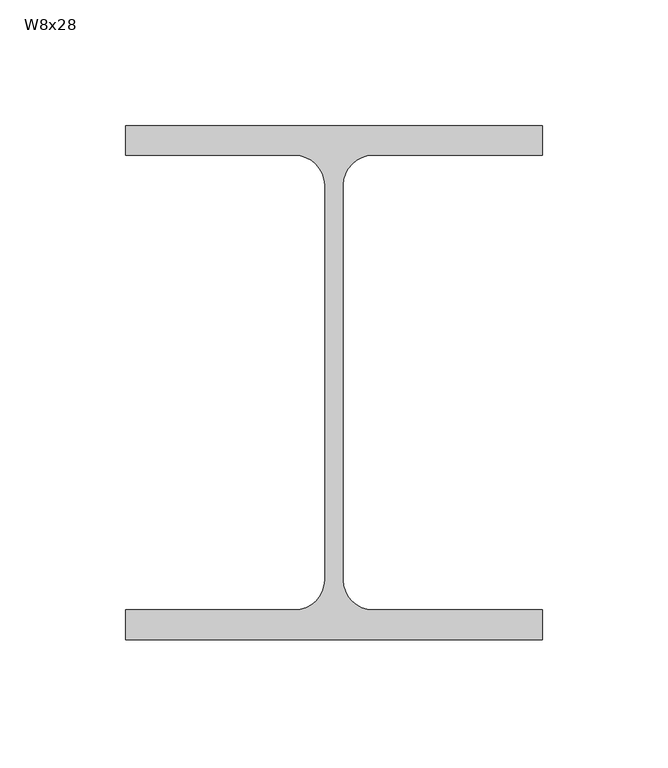
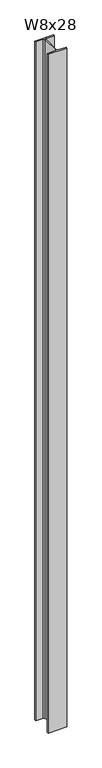
"""IFC4 building model written with IfcOpenShell, lengths in millimetres: column geometry, RME WF - Column : W8x28."""

import ifcopenshell
import ifcopenshell.guid

model = None  # the IFC model being written
_history = None  # IfcOwnerHistory: only IFC2X3 demands one
_inside = {}  # id of a spatial element -> (the spatial element, [elements in it])
_under = {}  # id of a project, library or spatial element -> (it, [spatial elements below it])
_declared = {}  # id of a project -> (the project, [libraries it declares])
_typed = {}  # id of a type object -> (the type object, [elements of that type])
_made_of = {}  # id of a material, layer set ... -> (it, [elements and type objects made of it])


def new_model(schema):
    """Start an empty IFC model of exactly this schema.

    Asked for "IFC4X3", IfcOpenShell would pick the latest addendum, in which some entities
    have other attributes; the version numbers below select the first issue.
    IFC2X3 requires an IfcOwnerHistory on every rooted entity: one is made here for all.
    """
    global model, _history
    if schema == "IFC4X3":
        model = ifcopenshell.file(schema_version=(4, 3, 0, 0))
    else:
        model = ifcopenshell.file(schema=schema)
    _inside.clear()
    _under.clear()
    _declared.clear()
    _typed.clear()
    _made_of.clear()
    _history = None
    if model.schema == "IFC2X3":
        org = make("IfcOrganization", Name="unknown")
        user = make(
            "IfcPersonAndOrganization",
            ThePerson=make("IfcPerson", FamilyName="unknown"),
            TheOrganization=org,
        )
        app = make(
            "IfcApplication",
            ApplicationDeveloper=org,
            Version="unknown",
            ApplicationFullName="unknown",
            ApplicationIdentifier="unknown",
        )
        _history = make(
            "IfcOwnerHistory",
            OwningUser=user,
            OwningApplication=app,
            ChangeAction="ADDED",
            CreationDate=0,
        )
    return model


def make(cls, **values):
    """One entity of the class cls with the attributes given. An attribute that is None is left unset."""
    return model.create_entity(
        cls, **{name: value for name, value in values.items() if value is not None}
    )


def rooted(cls, **values):
    """An entity with a GlobalId (a new one), such as an element, a storey or a relation."""
    return make(cls, GlobalId=ifcopenshell.guid.new(), OwnerHistory=_history, **values)


def si_unit(unit_type, name, prefix=None):
    """IfcSIUnit, for example si_unit("LENGTHUNIT", "METRE", prefix="MILLI")."""
    return make("IfcSIUnit", UnitType=unit_type, Prefix=prefix, Name=name)


def assignment(units):
    """IfcUnitAssignment: the units of a project."""
    return None if units is None else make("IfcUnitAssignment", Units=units)


def point(xyz):
    """IfcCartesianPoint."""
    return None if xyz is None else make("IfcCartesianPoint", Coordinates=xyz)


def direction(xyz):
    """IfcDirection."""
    return None if xyz is None else make("IfcDirection", DirectionRatios=xyz)


def frame(location, z_axis=None, x_axis=None):
    """IfcAxis2Placement3D, a coordinate frame: its origin and axes. An axis left out is left unset."""
    return make(
        "IfcAxis2Placement3D",
        Location=point(location),
        Axis=direction(z_axis),
        RefDirection=direction(x_axis),
    )


def frame_2d(location, x_axis=None):
    """IfcAxis2Placement2D, a coordinate frame in the plane: its origin and x axis."""
    return make(
        "IfcAxis2Placement2D", Location=point(location), RefDirection=direction(x_axis)
    )


def origin():
    """The frame at (0, 0, 0) with its axes left unset."""
    return frame((0.0, 0.0, 0.0))


def place(relative_to, where):
    """IfcLocalPlacement: puts the frame where relative to a parent placement (None: the world)."""
    return make(
        "IfcLocalPlacement", PlacementRelTo=relative_to, RelativePlacement=where
    )


def context(
    kind, dimensions, precision=None, world=None, true_north=None, identifier=None
):
    """IfcGeometricRepresentationContext, for example the 3D "Model" context."""
    return make(
        "IfcGeometricRepresentationContext",
        ContextIdentifier=identifier,
        ContextType=kind,
        CoordinateSpaceDimension=dimensions,
        Precision=precision,
        WorldCoordinateSystem=world,
        TrueNorth=true_north,
    )


def project(units=None, contexts=None):
    """IfcProject with its units and contexts."""
    return rooted(
        "IfcProject",
        Name="project",
        RepresentationContexts=contexts,
        UnitsInContext=assignment(units),
    )


def spatial(cls, under=None, at=None, **own):
    """A site, building, storey or space (cls), placed at a placement, below another one or the project."""
    s = rooted(cls, ObjectPlacement=at, **own)
    if under is not None:
        _under.setdefault(under.id(), (under, []))[1].append(s)
    return s


def polyline(points):
    """IfcPolyline through the points."""
    return make("IfcPolyline", Points=[point(p) for p in points])


def circle_curve(where, radius):
    """IfcCircle in the frame where."""
    return make("IfcCircle", Position=where, Radius=radius)


def trimmed(basis, trim1, trim2, sense, master):
    """IfcTrimmedCurve: the piece of a basis curve between two trims."""
    return make(
        "IfcTrimmedCurve",
        BasisCurve=basis,
        Trim1=trim1,
        Trim2=trim2,
        SenseAgreement=sense,
        MasterRepresentation=master,
    )


def segment(curve, same_sense, transition):
    """IfcCompositeCurveSegment."""
    return make(
        "IfcCompositeCurveSegment",
        Transition=transition,
        SameSense=same_sense,
        ParentCurve=curve,
    )


def composite_curve(segments, self_intersect=None):
    """IfcCompositeCurve: segments joined end to end."""
    return make("IfcCompositeCurve", Segments=segments, SelfIntersect=self_intersect)


def outline(outer, holes=None, kind="AREA"):
    """IfcArbitraryClosedProfileDef: a profile drawn as a closed curve; with holes, ...WithVoids."""
    if holes is None:
        return make("IfcArbitraryClosedProfileDef", ProfileType=kind, OuterCurve=outer)
    return make(
        "IfcArbitraryProfileDefWithVoids",
        ProfileType=kind,
        OuterCurve=outer,
        InnerCurves=holes,
    )


def extrude(swept, where, along, depth):
    """IfcExtrudedAreaSolid: the profile swept, set in the frame where, extruded along a direction by depth."""
    return make(
        "IfcExtrudedAreaSolid",
        SweptArea=swept,
        Position=where,
        ExtrudedDirection=direction(along),
        Depth=depth,
    )


def shape(context_of_items, identifier, shape_type, items):
    """IfcShapeRepresentation: the items that make up one representation, for example the "Body"."""
    return make(
        "IfcShapeRepresentation",
        ContextOfItems=context_of_items,
        RepresentationIdentifier=identifier,
        RepresentationType=shape_type,
        Items=items,
    )


def source(mapping_origin, context_of_items, identifier, shape_type, items):
    """IfcRepresentationMap: a shape defined once, which mapped items show again and again."""
    return make(
        "IfcRepresentationMap",
        MappingOrigin=mapping_origin,
        MappedRepresentation=shape(context_of_items, identifier, shape_type, items),
    )


def transform(
    local_origin,
    x_axis=None,
    y_axis=None,
    z_axis=None,
    scale=None,
    scale2=None,
    scale3=None,
    uniform=True,
):
    """IfcCartesianTransformationOperator3D, or its non-uniform kind. x_axis, y_axis, z_axis: its Axis1, 2, 3."""
    if uniform:
        return make(
            "IfcCartesianTransformationOperator3D",
            Axis1=direction(x_axis),
            Axis2=direction(y_axis),
            LocalOrigin=point(local_origin),
            Scale=scale,
            Axis3=direction(z_axis),
        )
    return make(
        "IfcCartesianTransformationOperator3DnonUniform",
        Axis1=direction(x_axis),
        Axis2=direction(y_axis),
        LocalOrigin=point(local_origin),
        Scale=scale,
        Axis3=direction(z_axis),
        Scale2=scale2,
        Scale3=scale3,
    )


def mapped(mapping_source, mapping_target):
    """IfcMappedItem: shows the shape of a source again, moved by a transform."""
    return make(
        "IfcMappedItem", MappingSource=mapping_source, MappingTarget=mapping_target
    )


def made_of(thing, what):
    """Note that an element or type object is made of a material, layer set ...; save() writes the relation."""
    if what is not None:
        _made_of.setdefault(what.id(), (what, []))[1].append(thing)
    return thing


def element(
    cls,
    number,
    at=None,
    inside=None,
    cuts=None,
    type_object=None,
    material=None,
    context=None,
    identifier="Body",
    shape_type=None,
    held_by="IfcProductDefinitionShape",
    body=None,
    shapes=None,
    **own,
):
    """One element of the class cls, such as IfcWall. Its Tag is "e" and its number.

    at: its placement. inside: the storey or other place that contains it. cuts: it is an
    opening in that element (IfcRelVoidsElement). A single representation is given by context,
    identifier, shape_type and body (its items); several are given by shapes. held_by: the class
    of the entity that holds the representations. save() writes the other relations.
    """
    e = rooted(cls, Tag="e%d" % number, ObjectPlacement=at, **own)
    if body is not None:
        shapes = [shape(context, identifier, shape_type, body)]
    if shapes is not None:
        e.Representation = make(held_by, Representations=shapes)
    if inside is not None:
        _inside.setdefault(inside.id(), (inside, []))[1].append(e)
    if cuts is not None:
        rooted(
            "IfcRelVoidsElement", RelatingBuildingElement=cuts, RelatedOpeningElement=e
        )
    if type_object is not None:
        _typed.setdefault(type_object.id(), (type_object, []))[1].append(e)
    return made_of(e, material)


def aggregate(whole, parts):
    """IfcRelAggregates: a whole, such as a stair, and the parts it consists of."""
    return rooted("IfcRelAggregates", RelatingObject=whole, RelatedObjects=parts)


def save(model, path):
    """Write the relations noted so far, then the file.

    IfcRelAggregates (storeys below a building ...), IfcRelContainedInSpatialStructure (elements
    in a storey), IfcRelDefinesByType, IfcRelAssociatesMaterial and IfcRelDeclares: one each for
    every whole, place, type object, material and project.
    """
    for whole, parts in _under.values():
        aggregate(whole, parts)
    for where, things in _inside.values():
        rooted(
            "IfcRelContainedInSpatialStructure",
            RelatedElements=things,
            RelatingStructure=where,
        )
    for kind, things in _typed.values():
        rooted("IfcRelDefinesByType", RelatedObjects=things, RelatingType=kind)
    for what, things in _made_of.values():
        rooted("IfcRelAssociatesMaterial", RelatedObjects=things, RelatingMaterial=what)
    for by, libraries in _declared.values():
        rooted("IfcRelDeclares", RelatingContext=by, RelatedDefinitions=libraries)
    model.write(path)


def w8x28_3524ed98(model_context):
    return source(origin(), model_context, "Body", "SweptSolid", [
        extrude(outline(composite_curve([segment(polyline([(83.058, 102.362), (83.058, 90.551), (15.621, 90.551)]), True, "CONTINUOUS"), segment(trimmed(circle_curve(frame_2d((15.621, 78.5495)), 12.0015), [point((15.621, 90.551))], [point((3.6195, 78.5495))], True, "CARTESIAN"), True, "CONTINUOUS"), segment(polyline([(3.6195, 78.5495), (3.6195, -78.5495)]), True, "CONTINUOUS"), segment(trimmed(circle_curve(frame_2d((15.621, -78.5495)), 12.0015), [point((3.6195, -78.5495))], [point((15.621, -90.551))], True, "CARTESIAN"), True, "CONTINUOUS"), segment(polyline([(15.621, -90.551), (83.058, -90.551), (83.058, -102.362), (-83.058, -102.362), (-83.058, -90.551), (-15.621, -90.551)]), True, "CONTINUOUS"), segment(trimmed(circle_curve(frame_2d((-15.621, -78.5495)), 12.0015), [point((-15.621, -90.551))], [point((-3.6195, -78.5495))], True, "CARTESIAN"), True, "CONTINUOUS"), segment(polyline([(-3.6195, -78.5495), (-3.6195, 78.5495)]), True, "CONTINUOUS"), segment(trimmed(circle_curve(frame_2d((-15.621, 78.5495)), 12.0015), [point((-3.6195, 78.5495))], [point((-15.621, 90.551))], True, "CARTESIAN"), True, "CONTINUOUS"), segment(polyline([(-15.621, 90.551), (-83.058, 90.551), (-83.058, 102.362), (83.058, 102.362)]), True, "CONTINUOUS")], self_intersect=False)), frame((0.0, 0.0, -304.8), z_axis=(0.0, 0.0, 1.0), x_axis=(1.0, 0.0, 0.0)), (0.0, 0.0, 1.0), 6394.45),
    ])


if __name__ == "__main__":
    model = new_model("IFC4")
    model_context = context("Model", 3, world=origin())
    ifc_project = project(units=[si_unit("LENGTHUNIT", "METRE", prefix="MILLI")], contexts=[model_context])
    site = spatial("IfcSite", under=ifc_project)
    building = spatial("IfcBuilding", under=site)
    placement = place(None, origin())
    w8x28_shape = w8x28_3524ed98(model_context)
    element("IfcColumn", 1, ObjectType="RME WF - Column : W8x28", at=placement, inside=building, context=model_context, shape_type="MappedRepresentation", body=[
        mapped(w8x28_shape, transform((0.0, 0.0, 0.0), x_axis=(1.0, 0.0, 0.0), y_axis=(0.0, 1.0, 0.0), z_axis=(0.0, 0.0, 1.0))),
    ])
    save(model, "model.ifc")

# Revit data of these elements
# Type "RME WF - Column : W8x28"
#   REINF TYPE [instance default] = ""
#   Nominal Size = "W16"
#   COL REMARKS [instance default] = ""
#   BP [instance default] = ""
#   Assembly Code = "B10"
#   W = 28
#   bf = 0' - 6.54"
#   d = 0' - 8.06"
#   k = 0' - 0 15/16"
#   kr = 0' - 0.4725"
#   tf = 0' - 0.465"
#   tw = 0' - 0.285"
#   A = 0.0572222 SF
#   Structural Material [instance default] = Metal - Steel - ASTM A992
# Element 1 (IfcColumn, "RME WF - Column : W8x28")
#   Materials on its faces: "Metal - Steel - ASTM A992"
# Materials
#   "Metal - Steel - ASTM A992": class "Metal", colour RGB 255 128 0, transparency 0
